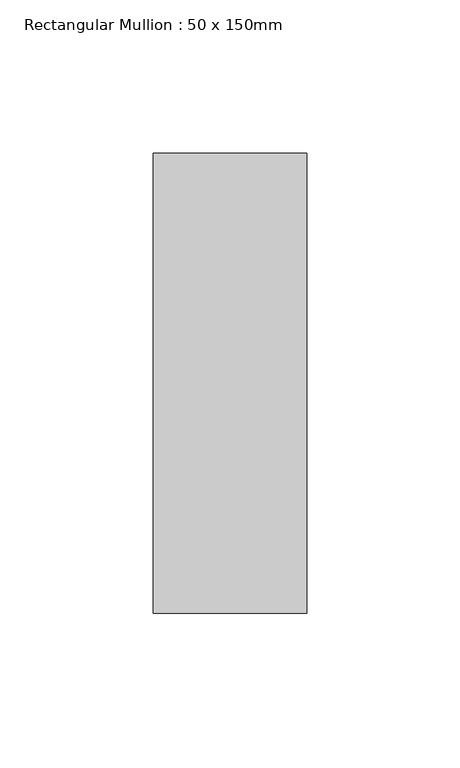
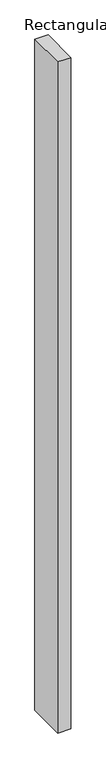
"""IFC4 building model written with IfcOpenShell, lengths in millimetres: member geometry, Rectangular Mullion : 50 x 150mm."""

import ifcopenshell
import ifcopenshell.guid

model = None  # the IFC model being written
_history = None  # IfcOwnerHistory: only IFC2X3 demands one
_inside = {}  # id of a spatial element -> (the spatial element, [elements in it])
_under = {}  # id of a project, library or spatial element -> (it, [spatial elements below it])
_declared = {}  # id of a project -> (the project, [libraries it declares])
_typed = {}  # id of a type object -> (the type object, [elements of that type])
_made_of = {}  # id of a material, layer set ... -> (it, [elements and type objects made of it])


def new_model(schema):
    """Start an empty IFC model of exactly this schema.

    Asked for "IFC4X3", IfcOpenShell would pick the latest addendum, in which some entities
    have other attributes; the version numbers below select the first issue.
    IFC2X3 requires an IfcOwnerHistory on every rooted entity: one is made here for all.
    """
    global model, _history
    if schema == "IFC4X3":
        model = ifcopenshell.file(schema_version=(4, 3, 0, 0))
    else:
        model = ifcopenshell.file(schema=schema)
    _inside.clear()
    _under.clear()
    _declared.clear()
    _typed.clear()
    _made_of.clear()
    _history = None
    if model.schema == "IFC2X3":
        org = make("IfcOrganization", Name="unknown")
        user = make(
            "IfcPersonAndOrganization",
            ThePerson=make("IfcPerson", FamilyName="unknown"),
            TheOrganization=org,
        )
        app = make(
            "IfcApplication",
            ApplicationDeveloper=org,
            Version="unknown",
            ApplicationFullName="unknown",
            ApplicationIdentifier="unknown",
        )
        _history = make(
            "IfcOwnerHistory",
            OwningUser=user,
            OwningApplication=app,
            ChangeAction="ADDED",
            CreationDate=0,
        )
    return model


def make(cls, **values):
    """One entity of the class cls with the attributes given. An attribute that is None is left unset."""
    return model.create_entity(
        cls, **{name: value for name, value in values.items() if value is not None}
    )


def rooted(cls, **values):
    """An entity with a GlobalId (a new one), such as an element, a storey or a relation."""
    return make(cls, GlobalId=ifcopenshell.guid.new(), OwnerHistory=_history, **values)


def si_unit(unit_type, name, prefix=None):
    """IfcSIUnit, for example si_unit("LENGTHUNIT", "METRE", prefix="MILLI")."""
    return make("IfcSIUnit", UnitType=unit_type, Prefix=prefix, Name=name)


def assignment(units):
    """IfcUnitAssignment: the units of a project."""
    return None if units is None else make("IfcUnitAssignment", Units=units)


def point(xyz):
    """IfcCartesianPoint."""
    return None if xyz is None else make("IfcCartesianPoint", Coordinates=xyz)


def direction(xyz):
    """IfcDirection."""
    return None if xyz is None else make("IfcDirection", DirectionRatios=xyz)


def frame(location, z_axis=None, x_axis=None):
    """IfcAxis2Placement3D, a coordinate frame: its origin and axes. An axis left out is left unset."""
    return make(
        "IfcAxis2Placement3D",
        Location=point(location),
        Axis=direction(z_axis),
        RefDirection=direction(x_axis),
    )


def origin():
    """The frame at (0, 0, 0) with its axes left unset."""
    return frame((0.0, 0.0, 0.0))


def place(relative_to, where):
    """IfcLocalPlacement: puts the frame where relative to a parent placement (None: the world)."""
    return make(
        "IfcLocalPlacement", PlacementRelTo=relative_to, RelativePlacement=where
    )


def context(
    kind, dimensions, precision=None, world=None, true_north=None, identifier=None
):
    """IfcGeometricRepresentationContext, for example the 3D "Model" context."""
    return make(
        "IfcGeometricRepresentationContext",
        ContextIdentifier=identifier,
        ContextType=kind,
        CoordinateSpaceDimension=dimensions,
        Precision=precision,
        WorldCoordinateSystem=world,
        TrueNorth=true_north,
    )


def project(units=None, contexts=None):
    """IfcProject with its units and contexts."""
    return rooted(
        "IfcProject",
        Name="project",
        RepresentationContexts=contexts,
        UnitsInContext=assignment(units),
    )


def spatial(cls, under=None, at=None, **own):
    """A site, building, storey or space (cls), placed at a placement, below another one or the project."""
    s = rooted(cls, ObjectPlacement=at, **own)
    if under is not None:
        _under.setdefault(under.id(), (under, []))[1].append(s)
    return s


def polyline(points):
    """IfcPolyline through the points."""
    return make("IfcPolyline", Points=[point(p) for p in points])


def outline(outer, holes=None, kind="AREA"):
    """IfcArbitraryClosedProfileDef: a profile drawn as a closed curve; with holes, ...WithVoids."""
    if holes is None:
        return make("IfcArbitraryClosedProfileDef", ProfileType=kind, OuterCurve=outer)
    return make(
        "IfcArbitraryProfileDefWithVoids",
        ProfileType=kind,
        OuterCurve=outer,
        InnerCurves=holes,
    )


def extrude(swept, where, along, depth):
    """IfcExtrudedAreaSolid: the profile swept, set in the frame where, extruded along a direction by depth."""
    return make(
        "IfcExtrudedAreaSolid",
        SweptArea=swept,
        Position=where,
        ExtrudedDirection=direction(along),
        Depth=depth,
    )


def shape(context_of_items, identifier, shape_type, items):
    """IfcShapeRepresentation: the items that make up one representation, for example the "Body"."""
    return make(
        "IfcShapeRepresentation",
        ContextOfItems=context_of_items,
        RepresentationIdentifier=identifier,
        RepresentationType=shape_type,
        Items=items,
    )


def source(mapping_origin, context_of_items, identifier, shape_type, items):
    """IfcRepresentationMap: a shape defined once, which mapped items show again and again."""
    return make(
        "IfcRepresentationMap",
        MappingOrigin=mapping_origin,
        MappedRepresentation=shape(context_of_items, identifier, shape_type, items),
    )


def transform(
    local_origin,
    x_axis=None,
    y_axis=None,
    z_axis=None,
    scale=None,
    scale2=None,
    scale3=None,
    uniform=True,
):
    """IfcCartesianTransformationOperator3D, or its non-uniform kind. x_axis, y_axis, z_axis: its Axis1, 2, 3."""
    if uniform:
        return make(
            "IfcCartesianTransformationOperator3D",
            Axis1=direction(x_axis),
            Axis2=direction(y_axis),
            LocalOrigin=point(local_origin),
            Scale=scale,
            Axis3=direction(z_axis),
        )
    return make(
        "IfcCartesianTransformationOperator3DnonUniform",
        Axis1=direction(x_axis),
        Axis2=direction(y_axis),
        LocalOrigin=point(local_origin),
        Scale=scale,
        Axis3=direction(z_axis),
        Scale2=scale2,
        Scale3=scale3,
    )


def mapped(mapping_source, mapping_target):
    """IfcMappedItem: shows the shape of a source again, moved by a transform."""
    return make(
        "IfcMappedItem", MappingSource=mapping_source, MappingTarget=mapping_target
    )


def made_of(thing, what):
    """Note that an element or type object is made of a material, layer set ...; save() writes the relation."""
    if what is not None:
        _made_of.setdefault(what.id(), (what, []))[1].append(thing)
    return thing


def element(
    cls,
    number,
    at=None,
    inside=None,
    cuts=None,
    type_object=None,
    material=None,
    context=None,
    identifier="Body",
    shape_type=None,
    held_by="IfcProductDefinitionShape",
    body=None,
    shapes=None,
    **own,
):
    """One element of the class cls, such as IfcWall. Its Tag is "e" and its number.

    at: its placement. inside: the storey or other place that contains it. cuts: it is an
    opening in that element (IfcRelVoidsElement). A single representation is given by context,
    identifier, shape_type and body (its items); several are given by shapes. held_by: the class
    of the entity that holds the representations. save() writes the other relations.
    """
    e = rooted(cls, Tag="e%d" % number, ObjectPlacement=at, **own)
    if body is not None:
        shapes = [shape(context, identifier, shape_type, body)]
    if shapes is not None:
        e.Representation = make(held_by, Representations=shapes)
    if inside is not None:
        _inside.setdefault(inside.id(), (inside, []))[1].append(e)
    if cuts is not None:
        rooted(
            "IfcRelVoidsElement", RelatingBuildingElement=cuts, RelatedOpeningElement=e
        )
    if type_object is not None:
        _typed.setdefault(type_object.id(), (type_object, []))[1].append(e)
    return made_of(e, material)


def aggregate(whole, parts):
    """IfcRelAggregates: a whole, such as a stair, and the parts it consists of."""
    return rooted("IfcRelAggregates", RelatingObject=whole, RelatedObjects=parts)


def save(model, path):
    """Write the relations noted so far, then the file.

    IfcRelAggregates (storeys below a building ...), IfcRelContainedInSpatialStructure (elements
    in a storey), IfcRelDefinesByType, IfcRelAssociatesMaterial and IfcRelDeclares: one each for
    every whole, place, type object, material and project.
    """
    for whole, parts in _under.values():
        aggregate(whole, parts)
    for where, things in _inside.values():
        rooted(
            "IfcRelContainedInSpatialStructure",
            RelatedElements=things,
            RelatingStructure=where,
        )
    for kind, things in _typed.values():
        rooted("IfcRelDefinesByType", RelatedObjects=things, RelatingType=kind)
    for what, things in _made_of.values():
        rooted("IfcRelAssociatesMaterial", RelatedObjects=things, RelatingMaterial=what)
    for by, libraries in _declared.values():
        rooted("IfcRelDeclares", RelatingContext=by, RelatedDefinitions=libraries)
    model.write(path)


def rectangular_mullion_50_x_150mm_cf0a7a0a(model_context):
    return source(origin(), model_context, "Body", "SweptSolid", [
        extrude(outline(polyline([(25.0, 75.0), (25.0, -75.0), (-25.0, -75.0), (-25.0, 75.0), (25.0, 75.0)])), frame((0.0, 0.0, -2700.0), z_axis=(0.0, 0.0, 1.0), x_axis=(1.0, 0.0, 0.0)), (0.0, 0.0, 1.0), 2700.0),
    ])


if __name__ == "__main__":
    model = new_model("IFC4")
    model_context = context("Model", 3, world=origin())
    ifc_project = project(units=[si_unit("LENGTHUNIT", "METRE", prefix="MILLI")], contexts=[model_context])
    site = spatial("IfcSite", under=ifc_project)
    building = spatial("IfcBuilding", under=site)
    placement = place(None, origin())
    rectangular_mullion_50_x_150mm_shape = rectangular_mullion_50_x_150mm_cf0a7a0a(model_context)
    element("IfcMember", 1, ObjectType="Rectangular Mullion : 50 x 150mm", at=placement, inside=building, context=model_context, shape_type="MappedRepresentation", body=[
        mapped(rectangular_mullion_50_x_150mm_shape, transform((0.0, 0.0, 0.0), x_axis=(1.0, 0.0, 0.0), y_axis=(0.0, 1.0, 0.0), z_axis=(0.0, 0.0, 1.0))),
    ])
    save(model, "model.ifc")

# Revit data of these elements
# Type "Rectangular Mullion : 50 x 150mm"
#   built-in parameter 1007304 = 0.492126 (stored number, unit not read)
#   built-in parameter 1007301 = 0.082021 (stored number, unit not read)
#   built-in parameter 1007300 = 0.082021 (stored number, unit not read)
# Element 1 (IfcMember, "Rectangular Mullion : 50 x 150mm")
#   Materials on its faces: "Metal - Aluminium"
# Materials
#   "Metal - Aluminium": class "Metal", colour RGB 247 247 247, transparency 0
